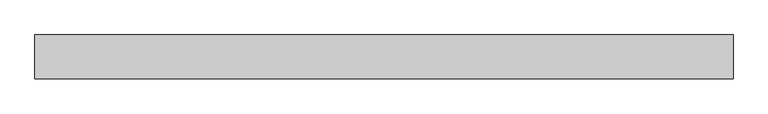
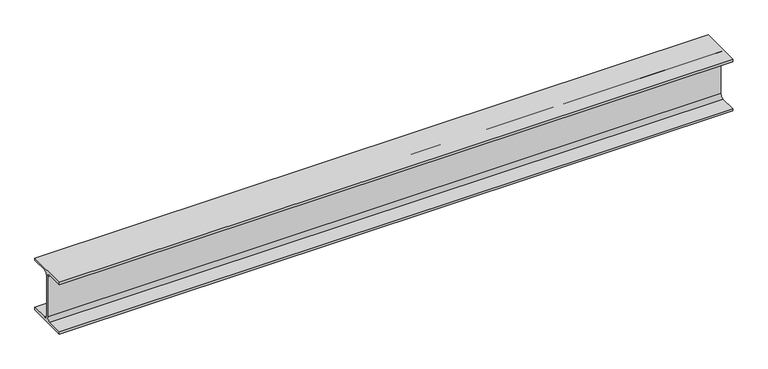
"""IFC4 building model written with IfcOpenShell, lengths in millimetres: beam geometry, 0912_Steel Framing_H-KSD3502 : H_SB_ASB_H-194x150x6x9."""

from ifc_helpers import new_model, si_unit, point, frame, frame_2d, origin, place, context, project, spatial, polyline, circle_curve, trimmed, segment, composite_curve, outline, extrude, source, transform, mapped, element, save


def beam_830b10b4(model_context):
    return source(origin(), model_context, "Body", "SweptSolid", [
        extrude(outline(composite_curve([segment(polyline([(75.0, -88.0), (75.0, -97.0), (-75.0, -97.0), (-75.0, -88.0), (-16.0, -88.0)]), True, "CONTINUOUS"), segment(trimmed(circle_curve(frame_2d((-16.0, -75.0)), 13.0), [point((-16.0, -88.0))], [point((-3.0, -75.0))], True, "CARTESIAN"), True, "CONTINUOUS"), segment(polyline([(-3.0, -75.0), (-3.0, 75.0)]), True, "CONTINUOUS"), segment(trimmed(circle_curve(frame_2d((-16.0, 75.0)), 13.0), [point((-3.0, 75.0))], [point((-16.0, 88.0))], True, "CARTESIAN"), True, "CONTINUOUS"), segment(polyline([(-16.0, 88.0), (-75.0, 88.0), (-75.0, 97.0), (75.0, 97.0), (75.0, 88.0), (16.0, 88.0)]), True, "CONTINUOUS"), segment(trimmed(circle_curve(frame_2d((16.0, 75.0)), 13.0), [point((16.0, 88.0))], [point((3.0, 75.0))], True, "CARTESIAN"), True, "CONTINUOUS"), segment(polyline([(3.0, 75.0), (3.0, -75.0)]), True, "CONTINUOUS"), segment(trimmed(circle_curve(frame_2d((16.0, -75.0)), 13.0), [point((3.0, -75.0))], [point((16.0, -88.0))], True, "CARTESIAN"), True, "CONTINUOUS"), segment(polyline([(16.0, -88.0), (75.0, -88.0)]), True, "CONTINUOUS")], self_intersect=False)), frame((-1520.0832263, 0.0, 0.0), z_axis=(1.0, 0.0, 0.0), x_axis=(0.0, 1.0, 0.0)), (0.0, 0.0, 1.0), 2387.3),
    ])


if __name__ == "__main__":
    model = new_model("IFC4")
    model_context = context("Model", 3, world=origin())
    ifc_project = project(units=[si_unit("LENGTHUNIT", "METRE", prefix="MILLI")], contexts=[model_context])
    site = spatial("IfcSite", under=ifc_project)
    building = spatial("IfcBuilding", under=site)
    placement = place(None, origin())
    beam_shape = beam_830b10b4(model_context)
    element("IfcBeam", 1, ObjectType="0912_Steel Framing_H-KSD3502 : H_SB_ASB_H-194x150x6x9", at=placement, inside=building, context=model_context, shape_type="MappedRepresentation", body=[
        mapped(beam_shape, transform((0.0, 0.0, 0.0), x_axis=(1.0, 0.0, 0.0), y_axis=(0.0, 1.0, 0.0), z_axis=(0.0, 0.0, 1.0))),
    ])
    save(model, "model.ifc")

# Revit data of these elements
# Type "0912_Steel Framing_H-KSD3502 : H_SB_ASB_H-194x150x6x9"
#   H_WM Code_1 = "S01AA002-00001 | Main Steel Structure Fabrication Work | Shelter/Building | Medium Steel - Standard (90KG/M>Weight≥30KG/M) | Material: (   )"
#   H_WM Code_2 = "S03AA028-00001 | Main Steel Structure Erection Work | Shelter/Building | Medium Steel (90KG/M>Weight≥30KG/M) | Material: (   )"
#   H_WM Code_3 = "S01AA010-00001 | Main Steel Structure Fabrication Work | Shelter/Building | Steel Painting/Coating | for Non-Fireproofed Steel Surface, Surface Preparation, Primer, Second & Final Coat | Material: (   )"
#   H_Q'ty Cal Type Tag = "SB-Q2"
#   Width = 15.0 cm
#   Web Thickness = 0.6 cm
#   Web Fillet = 1.3 cm
#   Warping Constant = 43316.0 cm⁶
#   W = 0
#   Torsional Moment of Inertia = 8.622 cm⁴
#   Section Area = 39.01 cm²
#   Plastic Modulus weak axis = 104.0 cm³
#   Plastic Modulus strong axis = 309.0 cm³
#   Perimeter = 0.95 m²/m
#   Nominal Weight = 30.60 kgf/m
#   Moment of Inertia weak axis = 507.00 cm⁴
#   Moment of Inertia strong axis = 2690.00 cm⁴
#   Height = 19.4 cm
#   Flange Thickness = 0.9 cm
#   Elastic Modulus weak axis = 67.6 cm³
#   Elastic Modulus strong axis = 277.0 cm³
#   Centroid Vertical = 9.7 cm
#   Centroid Horizontal = 7.5 cm
#   Ix = 26900000
#   Length [instance default] = 1.5240 m
#   Zx = 309000
#   b = 0.1500 m
#   h = 0.1940 m
#   r = 0.0130 m
#   s = 0.0060 m
#   t = 0.0090 m
#   A = 0.003901 m²
#   Structural Material [instance default] = Steel, 45-345
#   Assembly Code = ""
# Element 1 (IfcBeam, "0912_Steel Framing_H-KSD3502 : H_SB_ASB_H-194x150x6x9")
#   Structural Material = none
# Materials
#   "Steel, 45-345": class "Metal", colour RGB 189 187 185, transparency 0, Description = "Steel 345 MPa", Cost = 0
